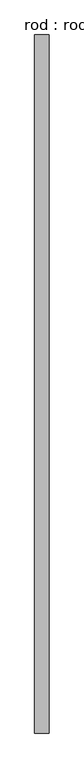
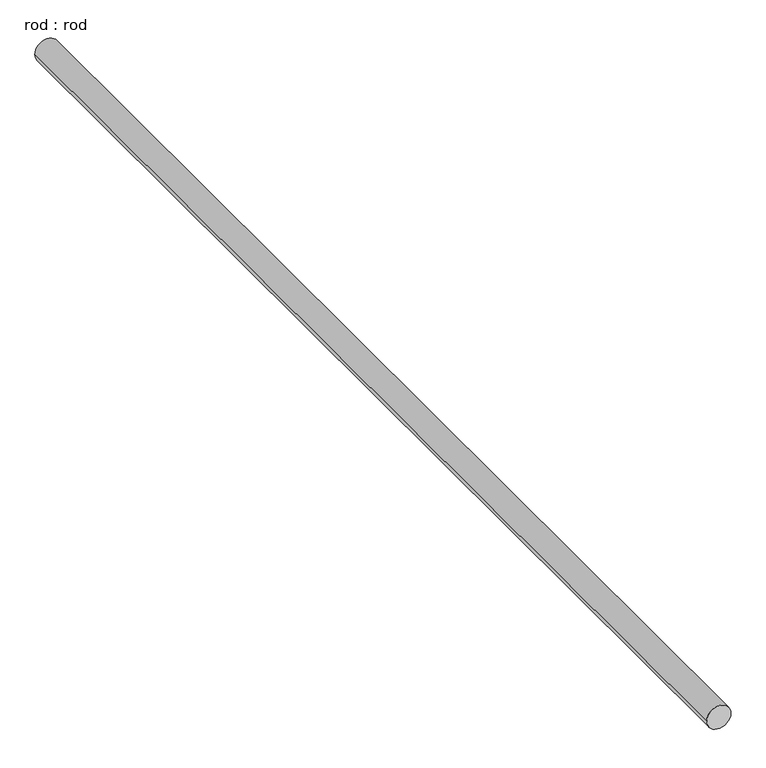
"""IFC4 building model written with IfcOpenShell, lengths in millimetres: proxy geometry, rod : rod."""

from ifc_helpers import new_model, si_unit, point, frame, frame_2d, origin, place, context, project, spatial, circle_curve, trimmed, segment, composite_curve, outline, extrude, source, transform, mapped, element, save


def rod_rod_318e75fa(model_context):
    return source(origin(), model_context, "Body", "SweptSolid", [
        extrude(outline(composite_curve([segment(trimmed(circle_curve(frame_2d((0.0108462, 0.0)), 200.0), [point((0.0108462, 200.0))], [point((0.0108462, -200.0))], False, "CARTESIAN"), True, "CONTINUOUS"), segment(trimmed(circle_curve(frame_2d((0.0108462, 0.0)), 200.0), [point((0.0108462, -200.0))], [point((0.0108462, 200.0))], False, "CARTESIAN"), True, "CONTINUOUS")], self_intersect=False)), frame((0.0, -5532.2713847, 0.0), z_axis=(0.0, 1.0, 0.0), x_axis=(0.0, 0.0, 1.0)), (0.0, 0.0, 1.0), 19250.0),
    ])


if __name__ == "__main__":
    model = new_model("IFC4")
    model_context = context("Model", 3, world=origin())
    ifc_project = project(units=[si_unit("LENGTHUNIT", "METRE", prefix="MILLI")], contexts=[model_context])
    site = spatial("IfcSite", under=ifc_project)
    building = spatial("IfcBuilding", under=site)
    placement = place(None, origin())
    rod_rod_shape = rod_rod_318e75fa(model_context)
    element("IfcBuildingElementProxy", 1, Name="rod : rod", ObjectType="rod : rod", at=placement, inside=building, context=model_context, shape_type="MappedRepresentation", body=[
        mapped(rod_rod_shape, transform((0.0, 0.0, 0.0), x_axis=(1.0, 0.0, 0.0), y_axis=(0.0, 1.0, 0.0), z_axis=(0.0, 0.0, 1.0))),
    ])
    save(model, "model.ifc")

# Revit data of these elements
# Type "rod : rod"
#   Default Elevation = 0
